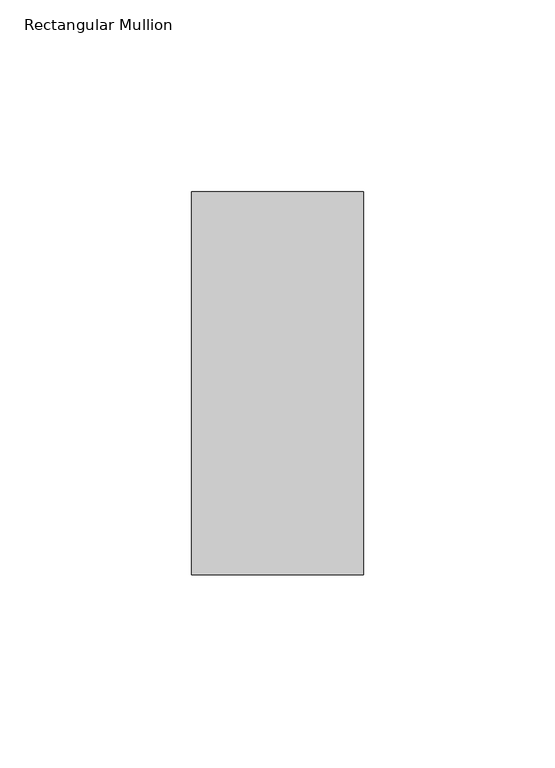
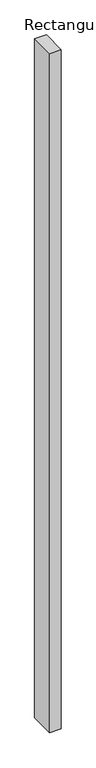
"""IFC4 building model written with IfcOpenShell, lengths in millimetres: member geometry, Rectangular Mullion : 알루미늄_Rectangular Cap_100 x 45."""

from ifc_helpers import new_model, si_unit, frame, origin, place, context, project, spatial, polyline, outline, extrude, source, transform, mapped, element, save


def rectangular_mullion_1b622e54(model_context):
    return source(origin(), model_context, "Body", "SweptSolid", [
        extrude(outline(polyline([(0.0, 50.0), (0.0, -50.0), (-45.0, -50.0), (-45.0, 50.0), (0.0, 50.0)])), frame((0.0, 0.0, -2777.0), z_axis=(0.0, 0.0, 1.0), x_axis=(1.0, 0.0, 0.0)), (0.0, 0.0, 1.0), 2777.0),
    ])


if __name__ == "__main__":
    model = new_model("IFC4")
    model_context = context("Model", 3, world=origin())
    ifc_project = project(units=[si_unit("LENGTHUNIT", "METRE", prefix="MILLI")], contexts=[model_context])
    site = spatial("IfcSite", under=ifc_project)
    building = spatial("IfcBuilding", under=site)
    placement = place(None, origin())
    rectangular_mullion_shape = rectangular_mullion_1b622e54(model_context)
    element("IfcMember", 1, ObjectType="Rectangular Mullion : 알루미늄_Rectangular Cap_100 x 45", at=placement, inside=building, context=model_context, shape_type="MappedRepresentation", body=[
        mapped(rectangular_mullion_shape, transform((0.0, 0.0, 0.0), x_axis=(1.0, 0.0, 0.0), y_axis=(0.0, 1.0, 0.0), z_axis=(0.0, 0.0, 1.0))),
    ])
    save(model, "model.ifc")

# Revit data of these elements
# Type "Rectangular Mullion : 알루미늄_Rectangular Cap_100 x 45"
#   built-in parameter 1007304 = 0.328084 (stored number, unit not read)
#   built-in parameter 1007301 = 0.0738189 (stored number, unit not read)
#   built-in parameter 1007300 = 0.0738189 (stored number, unit not read)
# Element 1 (IfcMember, "Rectangular Mullion : 알루미늄_Rectangular Cap_100 x 45")
#   Materials on its faces: "00_Metal_Stainless Steel"
# Materials
#   "00_Metal_Stainless Steel": class "Metal", colour RGB 148 148 148, transparency 0, Description = "Steel", Cost = 0
